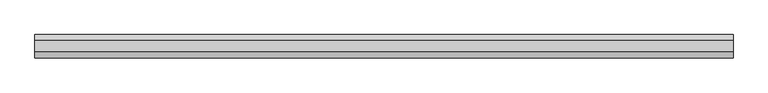
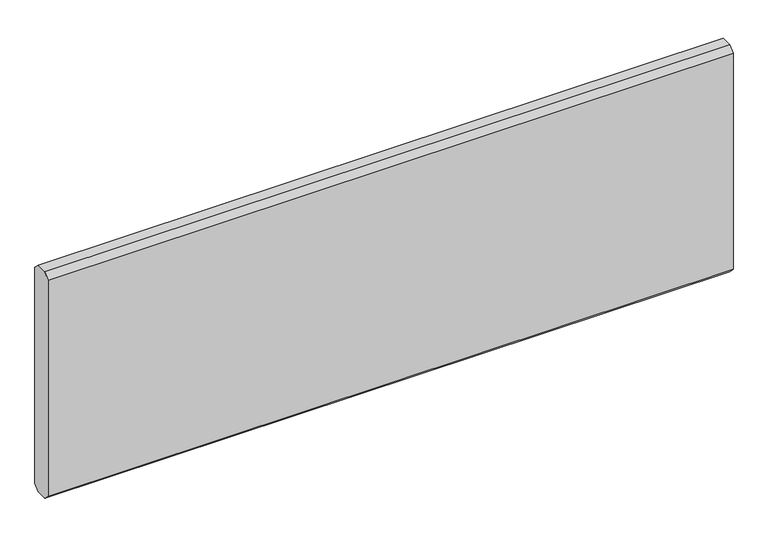
"""IFC4 building model written with IfcOpenShell, lengths in millimetres: proxy geometry, .RIPA : RIPA."""

from ifc_helpers import new_model, si_unit, frame, origin, place, context, project, spatial, polyline, outline, extrude, source, transform, mapped, element, save


def generic_models_d855a693(model_context):
    return source(origin(), model_context, "Body", "SweptSolid", [
        extrude(outline(polyline([(-12.5, 525.0), (12.5, 525.0), (25.0, 512.5), (25.0, 12.5), (12.5, 0.0), (-12.5, 0.0), (-25.0, 12.5), (-25.0, 512.5), (-12.5, 525.0)])), frame((-750.0, 0.0, 0.0), z_axis=(1.0, 0.0, 0.0), x_axis=(0.0, 1.0, 0.0)), (0.0, 0.0, 1.0), 1500.0),
    ])


if __name__ == "__main__":
    model = new_model("IFC4")
    model_context = context("Model", 3, world=origin())
    ifc_project = project(units=[si_unit("LENGTHUNIT", "METRE", prefix="MILLI")], contexts=[model_context])
    site = spatial("IfcSite", under=ifc_project)
    building = spatial("IfcBuilding", under=site)
    placement = place(None, origin())
    generic_models_shape = generic_models_d855a693(model_context)
    element("IfcBuildingElementProxy", 1, Name=".RIPA : RIPA", ObjectType=".RIPA : RIPA", at=placement, inside=building, context=model_context, shape_type="MappedRepresentation", body=[
        mapped(generic_models_shape, transform((0.0, 0.0, 0.0), x_axis=(1.0, 0.0, 0.0), y_axis=(0.0, 1.0, 0.0), z_axis=(0.0, 0.0, 1.0))),
    ])
    save(model, "model.ifc")

# Revit data of these elements
# Type ".RIPA : RIPA"
#   Ripa_largura [instance default] = 0.30 m
#   Ripa_espessura [instance default] = 0.025 m
#   Ripa_comprimento [instance default] = 0.80 m
#   Ripa_chanfo [instance default] = 0.00625 m
#   Ripa_material [instance default] = none
# Element 1 (IfcBuildingElementProxy, ".RIPA : RIPA")
#   Ripa_largura = 0.525 m
#   Ripa_espessura = 0.05 m
#   Ripa_comprimento = 1.50 m
#   Ripa_chanfo = 0.0125 m
#   Ripa_material = .MADEIRA_CEREJEIRA CLARO
#   Materials on its faces: ".MADEIRA_CEREJEIRA CLARO"
# Materials
#   ".MADEIRA_CEREJEIRA CLARO": class ".CC_MADEIRA REVEST.", colour RGB 233 182 144, transparency 0, Cost = 0
